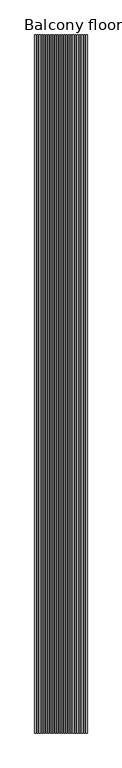
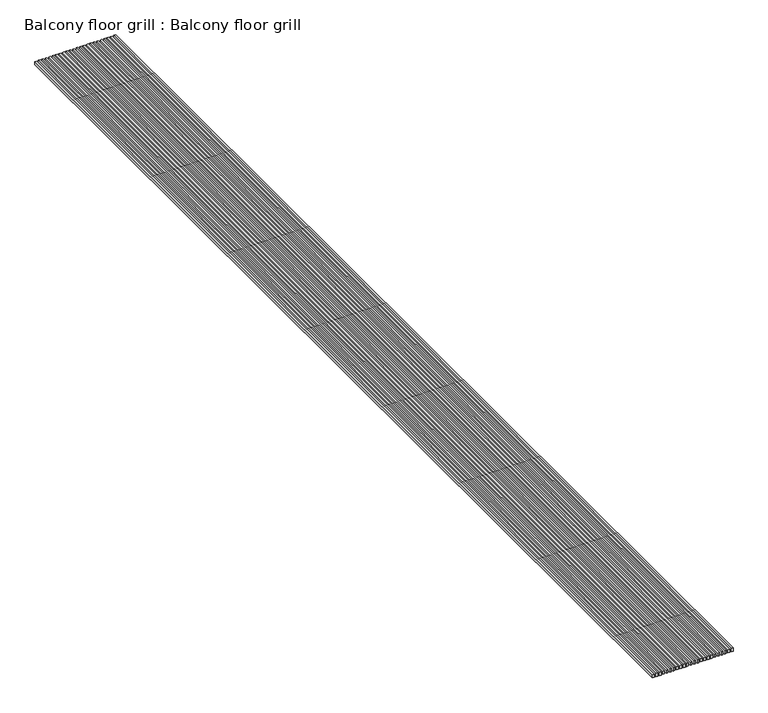
"""IFC4 building model written with IfcOpenShell, lengths in millimetres: proxy geometry, Balcony floor grill : Balcony floor grill."""

from ifc_helpers import new_model, si_unit, frame, origin, place, context, project, spatial, polyline, outline, extrude, source, transform, mapped, element, save


def balcony_floor_grill_balcony_floor_grill_0aae0050(model_context):
    return source(origin(), model_context, "Body", "SweptSolid", [
        extrude(outline(polyline([(25.4, -15836.9), (0.0, -15836.9), (0.0, 0.0), (25.4, 0.0), (25.4, -15836.9)])), frame((0.0, 0.0, -50.8), z_axis=(0.0, 0.0, 1.0), x_axis=(1.0, 0.0, 0.0)), (0.0, 0.0, 1.0), 50.8),
        extrude(outline(polyline([(76.2, -15836.9), (50.8, -15836.9), (50.8, 0.0), (76.2, 0.0), (76.2, -15836.9)])), frame((0.0, 0.0, -50.8), z_axis=(0.0, 0.0, 1.0), x_axis=(1.0, 0.0, 0.0)), (0.0, 0.0, 1.0), 50.8),
        extrude(outline(polyline([(127.0, -15836.9), (101.6, -15836.9), (101.6, 0.0), (127.0, 0.0), (127.0, -15836.9)])), frame((0.0, 0.0, -50.8), z_axis=(0.0, 0.0, 1.0), x_axis=(1.0, 0.0, 0.0)), (0.0, 0.0, 1.0), 50.8),
        extrude(outline(polyline([(177.8, -15836.9), (152.4, -15836.9), (152.4, 0.0), (177.8, 0.0), (177.8, -15836.9)])), frame((0.0, 0.0, -50.8), z_axis=(0.0, 0.0, 1.0), x_axis=(1.0, 0.0, 0.0)), (0.0, 0.0, 1.0), 50.8),
        extrude(outline(polyline([(228.6, -15836.9), (203.2, -15836.9), (203.2, 0.0), (228.6, 0.0), (228.6, -15836.9)])), frame((0.0, 0.0, -50.8), z_axis=(0.0, 0.0, 1.0), x_axis=(1.0, 0.0, 0.0)), (0.0, 0.0, 1.0), 50.8),
        extrude(outline(polyline([(279.4, -15836.9), (254.0, -15836.9), (254.0, 0.0), (279.4, 0.0), (279.4, -15836.9)])), frame((0.0, 0.0, -50.8), z_axis=(0.0, 0.0, 1.0), x_axis=(1.0, 0.0, 0.0)), (0.0, 0.0, 1.0), 50.8),
        extrude(outline(polyline([(330.2, -15836.9), (304.8, -15836.9), (304.8, 0.0), (330.2, 0.0), (330.2, -15836.9)])), frame((0.0, 0.0, -50.8), z_axis=(0.0, 0.0, 1.0), x_axis=(1.0, 0.0, 0.0)), (0.0, 0.0, 1.0), 50.8),
        extrude(outline(polyline([(381.0, -15836.9), (355.6, -15836.9), (355.6, 0.0), (381.0, 0.0), (381.0, -15836.9)])), frame((0.0, 0.0, -50.8), z_axis=(0.0, 0.0, 1.0), x_axis=(1.0, 0.0, 0.0)), (0.0, 0.0, 1.0), 50.8),
        extrude(outline(polyline([(431.8, -15836.9), (406.4, -15836.9), (406.4, 0.0), (431.8, 0.0), (431.8, -15836.9)])), frame((0.0, 0.0, -50.8), z_axis=(0.0, 0.0, 1.0), x_axis=(1.0, 0.0, 0.0)), (0.0, 0.0, 1.0), 50.8),
        extrude(outline(polyline([(482.6, -15836.9), (457.2, -15836.9), (457.2, 0.0), (482.6, 0.0), (482.6, -15836.9)])), frame((0.0, 0.0, -50.8), z_axis=(0.0, 0.0, 1.0), x_axis=(1.0, 0.0, 0.0)), (0.0, 0.0, 1.0), 50.8),
        extrude(outline(polyline([(533.4, -15836.9), (508.0, -15836.9), (508.0, 0.0), (533.4, 0.0), (533.4, -15836.9)])), frame((0.0, 0.0, -50.8), z_axis=(0.0, 0.0, 1.0), x_axis=(1.0, 0.0, 0.0)), (0.0, 0.0, 1.0), 50.8),
        extrude(outline(polyline([(584.2, -15836.9), (558.8, -15836.9), (558.8, 0.0), (584.2, 0.0), (584.2, -15836.9)])), frame((0.0, 0.0, -50.8), z_axis=(0.0, 0.0, 1.0), x_axis=(1.0, 0.0, 0.0)), (0.0, 0.0, 1.0), 50.8),
        extrude(outline(polyline([(635.0, -15836.9), (609.6, -15836.9), (609.6, 0.0), (635.0, 0.0), (635.0, -15836.9)])), frame((0.0, 0.0, -50.8), z_axis=(0.0, 0.0, 1.0), x_axis=(1.0, 0.0, 0.0)), (0.0, 0.0, 1.0), 50.8),
        extrude(outline(polyline([(685.8, -15836.9), (660.4, -15836.9), (660.4, 0.0), (685.8, 0.0), (685.8, -15836.9)])), frame((0.0, 0.0, -50.8), z_axis=(0.0, 0.0, 1.0), x_axis=(1.0, 0.0, 0.0)), (0.0, 0.0, 1.0), 50.8),
        extrude(outline(polyline([(736.6, -15836.9), (711.2, -15836.9), (711.2, 0.0), (736.6, 0.0), (736.6, -15836.9)])), frame((0.0, 0.0, -50.8), z_axis=(0.0, 0.0, 1.0), x_axis=(1.0, 0.0, 0.0)), (0.0, 0.0, 1.0), 50.8),
        extrude(outline(polyline([(787.4, -15836.9), (762.0, -15836.9), (762.0, 0.0), (787.4, 0.0), (787.4, -15836.9)])), frame((0.0, 0.0, -50.8), z_axis=(0.0, 0.0, 1.0), x_axis=(1.0, 0.0, 0.0)), (0.0, 0.0, 1.0), 50.8),
        extrude(outline(polyline([(838.2, -15836.9), (812.8, -15836.9), (812.8, 0.0), (838.2, 0.0), (838.2, -15836.9)])), frame((0.0, 0.0, -50.8), z_axis=(0.0, 0.0, 1.0), x_axis=(1.0, 0.0, 0.0)), (0.0, 0.0, 1.0), 50.8),
        extrude(outline(polyline([(889.0, -15836.9), (863.6, -15836.9), (863.6, 0.0), (889.0, 0.0), (889.0, -15836.9)])), frame((0.0, 0.0, -50.8), z_axis=(0.0, 0.0, 1.0), x_axis=(1.0, 0.0, 0.0)), (0.0, 0.0, 1.0), 50.8),
        extrude(outline(polyline([(939.8, -15836.9), (914.4, -15836.9), (914.4, 0.0), (939.8, 0.0), (939.8, -15836.9)])), frame((0.0, 0.0, -50.8), z_axis=(0.0, 0.0, 1.0), x_axis=(1.0, 0.0, 0.0)), (0.0, 0.0, 1.0), 50.8),
        extrude(outline(polyline([(990.6, -15836.9), (965.2, -15836.9), (965.2, 0.0), (990.6, 0.0), (990.6, -15836.9)])), frame((0.0, 0.0, -50.8), z_axis=(0.0, 0.0, 1.0), x_axis=(1.0, 0.0, 0.0)), (0.0, 0.0, 1.0), 50.8),
        extrude(outline(polyline([(1041.4, -15836.9), (1016.0, -15836.9), (1016.0, 0.0), (1041.4, 0.0), (1041.4, -15836.9)])), frame((0.0, 0.0, -50.8), z_axis=(0.0, 0.0, 1.0), x_axis=(1.0, 0.0, 0.0)), (0.0, 0.0, 1.0), 50.8),
        extrude(outline(polyline([(1092.2, -15836.9), (1066.8, -15836.9), (1066.8, 0.0), (1092.2, 0.0), (1092.2, -15836.9)])), frame((0.0, 0.0, -50.8), z_axis=(0.0, 0.0, 1.0), x_axis=(1.0, 0.0, 0.0)), (0.0, 0.0, 1.0), 50.8),
        extrude(outline(polyline([(1143.0, -15836.9), (1117.6, -15836.9), (1117.6, 0.0), (1143.0, 0.0), (1143.0, -15836.9)])), frame((0.0, 0.0, -50.8), z_axis=(0.0, 0.0, 1.0), x_axis=(1.0, 0.0, 0.0)), (0.0, 0.0, 1.0), 50.8),
        extrude(outline(polyline([(1193.8, -15836.9), (1168.4, -15836.9), (1168.4, 0.0), (1193.8, 0.0), (1193.8, -15836.9)])), frame((0.0, 0.0, -50.8), z_axis=(0.0, 0.0, 1.0), x_axis=(1.0, 0.0, 0.0)), (0.0, 0.0, 1.0), 50.8),
    ])


if __name__ == "__main__":
    model = new_model("IFC4")
    model_context = context("Model", 3, world=origin())
    ifc_project = project(units=[si_unit("LENGTHUNIT", "METRE", prefix="MILLI")], contexts=[model_context])
    site = spatial("IfcSite", under=ifc_project)
    building = spatial("IfcBuilding", under=site)
    placement = place(None, origin())
    balcony_floor_grill_balcony_floor_grill_shape = balcony_floor_grill_balcony_floor_grill_0aae0050(model_context)
    element("IfcBuildingElementProxy", 1, Name="Balcony floor grill : Balcony floor grill", ObjectType="Balcony floor grill : Balcony floor grill", at=placement, inside=building, context=model_context, shape_type="MappedRepresentation", body=[
        mapped(balcony_floor_grill_balcony_floor_grill_shape, transform((0.0, 0.0, 0.0), x_axis=(1.0, 0.0, 0.0), y_axis=(0.0, 1.0, 0.0), z_axis=(0.0, 0.0, 1.0))),
    ])
    save(model, "model.ifc")

# Revit data of these elements
# Type "Balcony floor grill : Balcony floor grill"
#   Length [instance default] = 1' - 0"
# Element 1 (IfcBuildingElementProxy, "Balcony floor grill : Balcony floor grill")
#   Length = 51' - 11 1/2"
